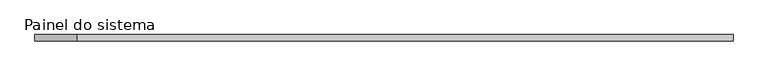
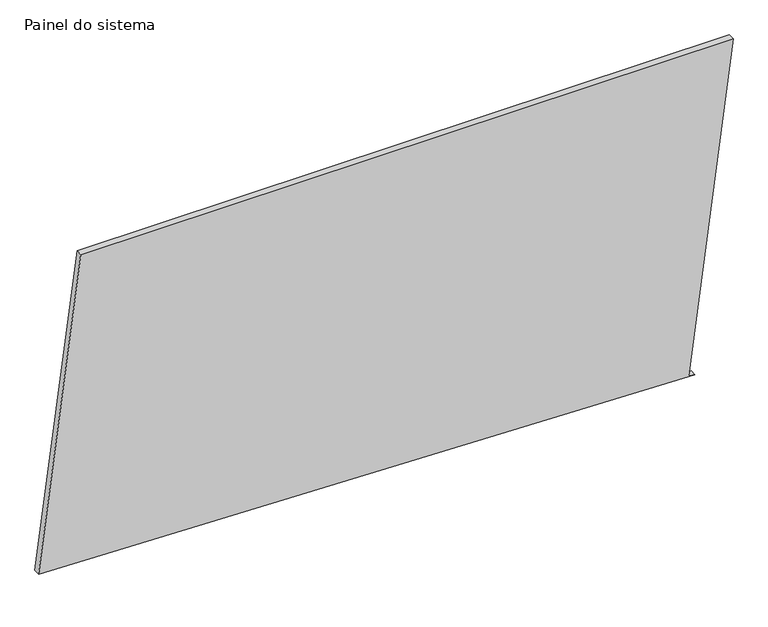
"""IFC4 building model written with IfcOpenShell, lengths in millimetres: plate geometry, Painel do sistema : Envidraçado."""

import ifcopenshell
import ifcopenshell.guid

model = None  # the IFC model being written
_history = None  # IfcOwnerHistory: only IFC2X3 demands one
_inside = {}  # id of a spatial element -> (the spatial element, [elements in it])
_under = {}  # id of a project, library or spatial element -> (it, [spatial elements below it])
_declared = {}  # id of a project -> (the project, [libraries it declares])
_typed = {}  # id of a type object -> (the type object, [elements of that type])
_made_of = {}  # id of a material, layer set ... -> (it, [elements and type objects made of it])


def new_model(schema):
    """Start an empty IFC model of exactly this schema.

    Asked for "IFC4X3", IfcOpenShell would pick the latest addendum, in which some entities
    have other attributes; the version numbers below select the first issue.
    IFC2X3 requires an IfcOwnerHistory on every rooted entity: one is made here for all.
    """
    global model, _history
    if schema == "IFC4X3":
        model = ifcopenshell.file(schema_version=(4, 3, 0, 0))
    else:
        model = ifcopenshell.file(schema=schema)
    _inside.clear()
    _under.clear()
    _declared.clear()
    _typed.clear()
    _made_of.clear()
    _history = None
    if model.schema == "IFC2X3":
        org = make("IfcOrganization", Name="unknown")
        user = make(
            "IfcPersonAndOrganization",
            ThePerson=make("IfcPerson", FamilyName="unknown"),
            TheOrganization=org,
        )
        app = make(
            "IfcApplication",
            ApplicationDeveloper=org,
            Version="unknown",
            ApplicationFullName="unknown",
            ApplicationIdentifier="unknown",
        )
        _history = make(
            "IfcOwnerHistory",
            OwningUser=user,
            OwningApplication=app,
            ChangeAction="ADDED",
            CreationDate=0,
        )
    return model


def make(cls, **values):
    """One entity of the class cls with the attributes given. An attribute that is None is left unset."""
    return model.create_entity(
        cls, **{name: value for name, value in values.items() if value is not None}
    )


def rooted(cls, **values):
    """An entity with a GlobalId (a new one), such as an element, a storey or a relation."""
    return make(cls, GlobalId=ifcopenshell.guid.new(), OwnerHistory=_history, **values)


def si_unit(unit_type, name, prefix=None):
    """IfcSIUnit, for example si_unit("LENGTHUNIT", "METRE", prefix="MILLI")."""
    return make("IfcSIUnit", UnitType=unit_type, Prefix=prefix, Name=name)


def assignment(units):
    """IfcUnitAssignment: the units of a project."""
    return None if units is None else make("IfcUnitAssignment", Units=units)


def point(xyz):
    """IfcCartesianPoint."""
    return None if xyz is None else make("IfcCartesianPoint", Coordinates=xyz)


def direction(xyz):
    """IfcDirection."""
    return None if xyz is None else make("IfcDirection", DirectionRatios=xyz)


def frame(location, z_axis=None, x_axis=None):
    """IfcAxis2Placement3D, a coordinate frame: its origin and axes. An axis left out is left unset."""
    return make(
        "IfcAxis2Placement3D",
        Location=point(location),
        Axis=direction(z_axis),
        RefDirection=direction(x_axis),
    )


def origin():
    """The frame at (0, 0, 0) with its axes left unset."""
    return frame((0.0, 0.0, 0.0))


def place(relative_to, where):
    """IfcLocalPlacement: puts the frame where relative to a parent placement (None: the world)."""
    return make(
        "IfcLocalPlacement", PlacementRelTo=relative_to, RelativePlacement=where
    )


def context(
    kind, dimensions, precision=None, world=None, true_north=None, identifier=None
):
    """IfcGeometricRepresentationContext, for example the 3D "Model" context."""
    return make(
        "IfcGeometricRepresentationContext",
        ContextIdentifier=identifier,
        ContextType=kind,
        CoordinateSpaceDimension=dimensions,
        Precision=precision,
        WorldCoordinateSystem=world,
        TrueNorth=true_north,
    )


def project(units=None, contexts=None):
    """IfcProject with its units and contexts."""
    return rooted(
        "IfcProject",
        Name="project",
        RepresentationContexts=contexts,
        UnitsInContext=assignment(units),
    )


def spatial(cls, under=None, at=None, **own):
    """A site, building, storey or space (cls), placed at a placement, below another one or the project."""
    s = rooted(cls, ObjectPlacement=at, **own)
    if under is not None:
        _under.setdefault(under.id(), (under, []))[1].append(s)
    return s


def polyline(points):
    """IfcPolyline through the points."""
    return make("IfcPolyline", Points=[point(p) for p in points])


def outline(outer, holes=None, kind="AREA"):
    """IfcArbitraryClosedProfileDef: a profile drawn as a closed curve; with holes, ...WithVoids."""
    if holes is None:
        return make("IfcArbitraryClosedProfileDef", ProfileType=kind, OuterCurve=outer)
    return make(
        "IfcArbitraryProfileDefWithVoids",
        ProfileType=kind,
        OuterCurve=outer,
        InnerCurves=holes,
    )


def extrude(swept, where, along, depth):
    """IfcExtrudedAreaSolid: the profile swept, set in the frame where, extruded along a direction by depth."""
    return make(
        "IfcExtrudedAreaSolid",
        SweptArea=swept,
        Position=where,
        ExtrudedDirection=direction(along),
        Depth=depth,
    )


def shape(context_of_items, identifier, shape_type, items):
    """IfcShapeRepresentation: the items that make up one representation, for example the "Body"."""
    return make(
        "IfcShapeRepresentation",
        ContextOfItems=context_of_items,
        RepresentationIdentifier=identifier,
        RepresentationType=shape_type,
        Items=items,
    )


def source(mapping_origin, context_of_items, identifier, shape_type, items):
    """IfcRepresentationMap: a shape defined once, which mapped items show again and again."""
    return make(
        "IfcRepresentationMap",
        MappingOrigin=mapping_origin,
        MappedRepresentation=shape(context_of_items, identifier, shape_type, items),
    )


def transform(
    local_origin,
    x_axis=None,
    y_axis=None,
    z_axis=None,
    scale=None,
    scale2=None,
    scale3=None,
    uniform=True,
):
    """IfcCartesianTransformationOperator3D, or its non-uniform kind. x_axis, y_axis, z_axis: its Axis1, 2, 3."""
    if uniform:
        return make(
            "IfcCartesianTransformationOperator3D",
            Axis1=direction(x_axis),
            Axis2=direction(y_axis),
            LocalOrigin=point(local_origin),
            Scale=scale,
            Axis3=direction(z_axis),
        )
    return make(
        "IfcCartesianTransformationOperator3DnonUniform",
        Axis1=direction(x_axis),
        Axis2=direction(y_axis),
        LocalOrigin=point(local_origin),
        Scale=scale,
        Axis3=direction(z_axis),
        Scale2=scale2,
        Scale3=scale3,
    )


def mapped(mapping_source, mapping_target):
    """IfcMappedItem: shows the shape of a source again, moved by a transform."""
    return make(
        "IfcMappedItem", MappingSource=mapping_source, MappingTarget=mapping_target
    )


def made_of(thing, what):
    """Note that an element or type object is made of a material, layer set ...; save() writes the relation."""
    if what is not None:
        _made_of.setdefault(what.id(), (what, []))[1].append(thing)
    return thing


def element(
    cls,
    number,
    at=None,
    inside=None,
    cuts=None,
    type_object=None,
    material=None,
    context=None,
    identifier="Body",
    shape_type=None,
    held_by="IfcProductDefinitionShape",
    body=None,
    shapes=None,
    **own,
):
    """One element of the class cls, such as IfcWall. Its Tag is "e" and its number.

    at: its placement. inside: the storey or other place that contains it. cuts: it is an
    opening in that element (IfcRelVoidsElement). A single representation is given by context,
    identifier, shape_type and body (its items); several are given by shapes. held_by: the class
    of the entity that holds the representations. save() writes the other relations.
    """
    e = rooted(cls, Tag="e%d" % number, ObjectPlacement=at, **own)
    if body is not None:
        shapes = [shape(context, identifier, shape_type, body)]
    if shapes is not None:
        e.Representation = make(held_by, Representations=shapes)
    if inside is not None:
        _inside.setdefault(inside.id(), (inside, []))[1].append(e)
    if cuts is not None:
        rooted(
            "IfcRelVoidsElement", RelatingBuildingElement=cuts, RelatedOpeningElement=e
        )
    if type_object is not None:
        _typed.setdefault(type_object.id(), (type_object, []))[1].append(e)
    return made_of(e, material)


def aggregate(whole, parts):
    """IfcRelAggregates: a whole, such as a stair, and the parts it consists of."""
    return rooted("IfcRelAggregates", RelatingObject=whole, RelatedObjects=parts)


def save(model, path):
    """Write the relations noted so far, then the file.

    IfcRelAggregates (storeys below a building ...), IfcRelContainedInSpatialStructure (elements
    in a storey), IfcRelDefinesByType, IfcRelAssociatesMaterial and IfcRelDeclares: one each for
    every whole, place, type object, material and project.
    """
    for whole, parts in _under.values():
        aggregate(whole, parts)
    for where, things in _inside.values():
        rooted(
            "IfcRelContainedInSpatialStructure",
            RelatedElements=things,
            RelatingStructure=where,
        )
    for kind, things in _typed.values():
        rooted("IfcRelDefinesByType", RelatedObjects=things, RelatingType=kind)
    for what, things in _made_of.values():
        rooted("IfcRelAssociatesMaterial", RelatedObjects=things, RelatingMaterial=what)
    for by, libraries in _declared.values():
        rooted("IfcRelDeclares", RelatingContext=by, RelatedDefinitions=libraries)
    model.write(path)


def painel_do_sistema_aac3b773(model_context):
    return source(origin(), model_context, "Body", "SweptSolid", [
        extrude(outline(polyline([(0.0, 1217.1138109), (3.2380023, 1192.3243909), (1346.18807, 1367.7409747), (1346.18807, -1201.5294625), (73.7099684, -1367.7409747), (0.0, 1217.1138109)])), frame((0.0, 24.5, 0.0), z_axis=(0.0, 1.0, 0.0), x_axis=(0.0, 0.0, 1.0)), (0.0, 0.0, 1.0), 25.0),
    ])


if __name__ == "__main__":
    model = new_model("IFC4")
    model_context = context("Model", 3, world=origin())
    ifc_project = project(units=[si_unit("LENGTHUNIT", "METRE", prefix="MILLI")], contexts=[model_context])
    site = spatial("IfcSite", under=ifc_project)
    building = spatial("IfcBuilding", under=site)
    placement = place(None, origin())
    painel_do_sistema_shape = painel_do_sistema_aac3b773(model_context)
    element("IfcPlate", 1, ObjectType="Painel do sistema : Envidraçado", at=placement, inside=building, context=model_context, shape_type="MappedRepresentation", body=[
        mapped(painel_do_sistema_shape, transform((0.0, 0.0, 0.0), x_axis=(1.0, 0.0, 0.0), y_axis=(0.0, 1.0, 0.0), z_axis=(0.0, 0.0, 1.0))),
    ])
    save(model, "model.ifc")

# Revit data of these elements
# Type "Painel do sistema : Envidraçado"
#   Construction Type Id = "GSP4R"
#   Analytic Construction = "Vidraça única Pilkington 1/8 pol"
#   Visual Light Transmittance = 0.9
#   Solar Heat Gain Coefficient = 0.86
#   Heat Transfer Coefficient (U) = 6.7069 W/(m²·K)
# Element 1 (IfcPlate, "Painel do sistema : Envidraçado")
#   Materials on its faces: "Vidro"
# Materials
#   "Vidro": class "Vidro", colour RGB 0 128 192, transparency 0.9, Description = "Vidro de sílica", Cost = 0
